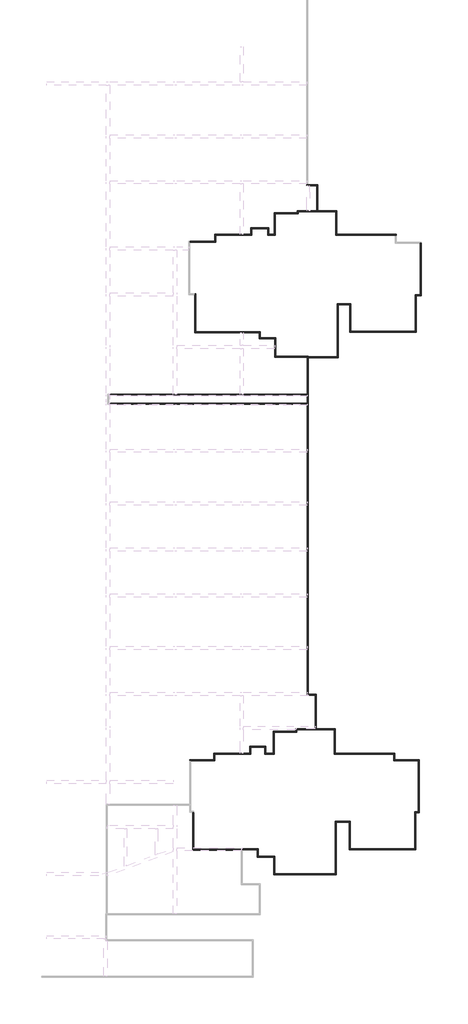
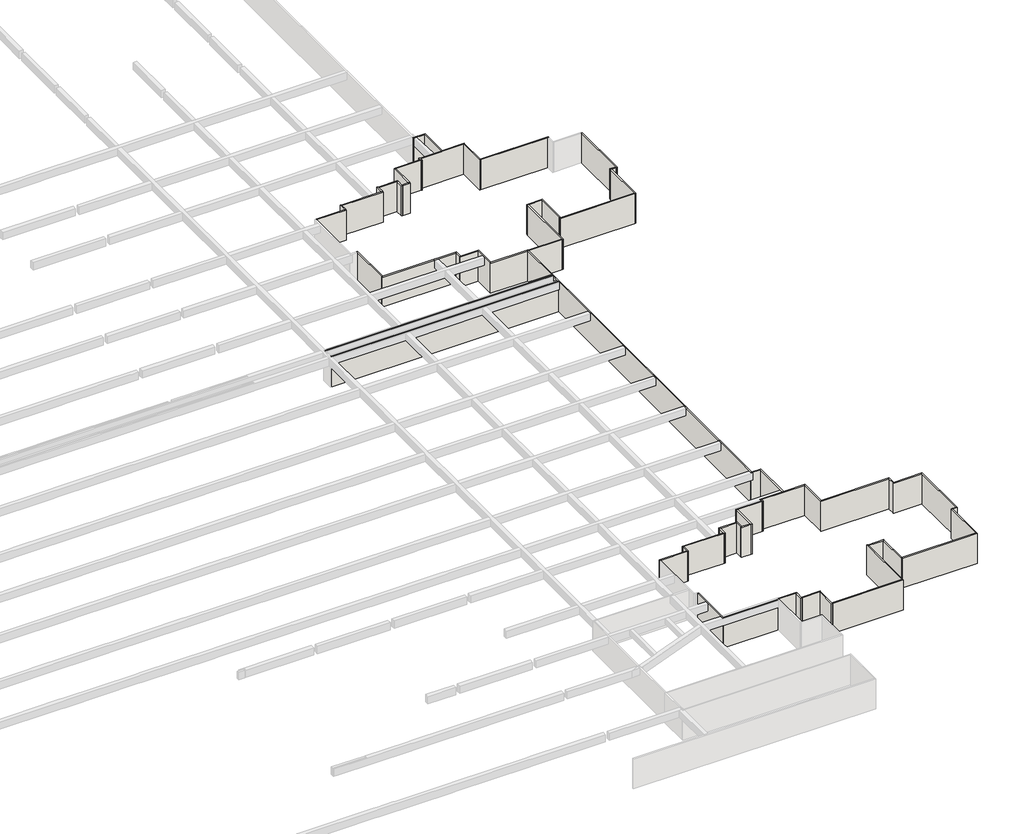
# One storey, part 5 of 14: 63 walls.
"""IFC4 building model written with IfcOpenShell, lengths in millimetres."""

from ifc_helpers import new_model, si_unit, origin, origin_with_axes, place, context, project, spatial, polyline, outline, extrude, faceted_brep, element, save

model = new_model("IFC4")

# Units and contexts
model_context = context("Model", 3, world=origin())
ifc_project = project(units=[si_unit("LENGTHUNIT", "METRE", prefix="MILLI")], contexts=[model_context])

# Site, building, storey
site = spatial("IfcSite", under=ifc_project)
building = spatial("IfcBuilding", under=site)
storey = spatial("IfcBuildingStorey", under=building, Name="户型图", Elevation=0.0)

# Walls
placement = place(None, origin())
element("IfcWall", 1, ObjectType="所有墙体", at=placement, inside=storey, context=model_context, shape_type="Brep", body=[
    faceted_brep([(-506007.6529952, -182584.2232736, 0.0), (-504227.6529952, -182584.2232736, 0.0), (-504107.6529952, -182584.2232736, 0.0), (-504107.6529952, -182584.2232736, 3300.0), (-504227.6529952, -182584.2232736, 3300.0), (-506007.6529952, -182584.2232736, 3300.0), (-506007.6529952, -182464.2232736, 0.0), (-506007.6529952, -182464.2232736, 3300.0), (-504107.6529952, -182464.2232736, 3300.0), (-504107.6529952, -182464.2232736, 0.0)], [[[0, 1, 2, 3, 4, 5]], [[6, 7, 8, 9]], [[2, 1, 0, 6, 9]], [[5, 4, 3, 8, 7]], [[0, 5, 7, 6]], [[3, 2, 9, 8]]]),
])
element("IfcWall", 2, ObjectType="所有墙体", at=placement, inside=storey, context=model_context, shape_type="Brep", body=[
    faceted_brep([(-504227.6529952, -182584.2232736, 0.0), (-504227.6529952, -183484.2232736, 0.0), (-504227.6529952, -183484.2232736, 3300.0), (-504227.6529952, -182584.2232736, 3300.0), (-504107.6529952, -182584.2232736, 0.0), (-504107.6529952, -182584.2232736, 3300.0), (-504107.6529952, -183364.2232736, 3300.0), (-504107.6529952, -183484.2232736, 3300.0), (-504107.6529952, -183484.2232736, 0.0), (-504107.6529952, -183364.2232736, 0.0)], [[[0, 1, 2, 3]], [[4, 5, 6, 7, 8, 9]], [[1, 0, 4, 9, 8]], [[3, 2, 7, 6, 5]], [[0, 3, 5, 4]], [[2, 1, 8, 7]]]),
])
element("IfcWall", 3, ObjectType="所有墙体", at=placement, inside=storey, context=model_context, shape_type="Brep", body=[
    faceted_brep([(-504107.6529952, -183484.2232736, 0.0), (-502261.0765844, -183484.2232736, 0.0), (-502141.0765844, -183484.2232736, 0.0), (-502141.0765844, -183484.2232736, 3300.0), (-502261.0765844, -183484.2232736, 3300.0), (-504107.6529952, -183484.2232736, 3300.0), (-504107.6529952, -183364.2232736, 0.0), (-504107.6529952, -183364.2232736, 3300.0), (-502141.0765844, -183364.2232736, 3300.0), (-502141.0765844, -183364.2232736, 0.0)], [[[0, 1, 2, 3, 4, 5]], [[6, 7, 8, 9]], [[2, 1, 0, 6, 9]], [[5, 4, 3, 8, 7]], [[0, 5, 7, 6]], [[3, 2, 9, 8]]]),
])
element("IfcWall", 4, ObjectType="所有墙体", at=placement, inside=storey, context=model_context, shape_type="Brep", body=[
    faceted_brep([(-502261.0765844, -183484.2232736, 0.0), (-502261.0765844, -185595.7483417, 0.0), (-502261.0765844, -185595.7483417, 3300.0), (-502261.0765844, -183484.2232736, 3300.0), (-502141.0765844, -183484.2232736, 0.0), (-502141.0765844, -183484.2232736, 3300.0), (-502141.0765844, -185475.7483417, 3300.0), (-502141.0765844, -185595.7483417, 3300.0), (-502141.0765844, -185595.7483417, 0.0), (-502141.0765844, -185475.7483417, 0.0)], [[[0, 1, 2, 3]], [[4, 5, 6, 7, 8, 9]], [[1, 0, 4, 9, 8]], [[3, 2, 7, 6, 5]], [[0, 3, 5, 4]], [[2, 1, 8, 7]]]),
])
element("IfcWall", 5, ObjectType="所有墙体", at=placement, inside=storey, context=model_context, shape_type="Brep", body=[
    faceted_brep([(-502141.0765844, -185595.7483417, 0.0), (-494747.3304181, -185595.7483417, 0.0), (-494747.3304181, -185595.7483417, 3300.0), (-502141.0765844, -185595.7483417, 3300.0), (-502141.0765844, -185475.7483417, 0.0), (-502141.0765844, -185475.7483417, 3300.0), (-494867.3304181, -185475.7483417, 3300.0), (-494747.3304181, -185475.7483417, 3300.0), (-494747.3304181, -185475.7483417, 0.0), (-494867.3304181, -185475.7483417, 0.0)], [[[0, 1, 2, 3]], [[4, 5, 6, 7, 8, 9]], [[1, 0, 4, 9, 8]], [[3, 2, 7, 6, 5]], [[0, 3, 5, 4]], [[2, 1, 8, 7]]]),
])
element("IfcWall", 6, ObjectType="所有墙体", at=placement, inside=storey, context=model_context, shape_type="Brep", body=[
    faceted_brep([(-494747.3304181, -185475.7483417, 0.0), (-494747.3304181, -179317.7334824, 0.0), (-494747.3304181, -179197.7334824, 0.0), (-494747.3304181, -179197.7334824, 3300.0), (-494747.3304181, -179317.7334824, 3300.0), (-494747.3304181, -185475.7483417, 3300.0), (-494867.3304181, -185475.7483417, 0.0), (-494867.3304181, -185475.7483417, 3300.0), (-494867.3304181, -179197.7334824, 3300.0), (-494867.3304181, -179197.7334824, 0.0)], [[[0, 1, 2, 3, 4, 5]], [[6, 7, 8, 9]], [[2, 1, 0, 6, 9]], [[5, 4, 3, 8, 7]], [[0, 5, 7, 6]], [[3, 2, 9, 8]]]),
])
element("IfcWall", 7, ObjectType="所有墙体", at=placement, inside=storey, context=model_context, shape_type="Brep", body=[
    faceted_brep([(-494747.3304181, -179317.7334824, 0.0), (-493248.6319968, -179317.7334824, 0.0), (-493128.6319968, -179317.7334824, 0.0), (-493128.6319968, -179317.7334824, 3300.0), (-493248.6319968, -179317.7334824, 3300.0), (-494747.3304181, -179317.7334824, 3300.0), (-494747.3304181, -179197.7334824, 0.0), (-494747.3304181, -179197.7334824, 3300.0), (-493128.6319968, -179197.7334824, 3300.0), (-493128.6319968, -179197.7334824, 0.0)], [[[0, 1, 2, 3, 4, 5]], [[6, 7, 8, 9]], [[2, 1, 0, 6, 9]], [[5, 4, 3, 8, 7]], [[0, 5, 7, 6]], [[3, 2, 9, 8]]]),
])
element("IfcWall", 8, ObjectType="所有墙体", at=placement, inside=storey, context=model_context, shape_type="Brep", body=[
    faceted_brep([(-493248.6319968, -179317.7334824, 0.0), (-493248.6319968, -182584.2232736, 0.0), (-493248.6319968, -182584.2232736, 3300.0), (-493248.6319968, -179317.7334824, 3300.0), (-493128.6319968, -179317.7334824, 0.0), (-493128.6319968, -179317.7334824, 3300.0), (-493128.6319968, -182464.2232736, 3300.0), (-493128.6319968, -182584.2232736, 3300.0), (-493128.6319968, -182584.2232736, 0.0), (-493128.6319968, -182464.2232736, 0.0)], [[[0, 1, 2, 3]], [[4, 5, 6, 7, 8, 9]], [[1, 0, 4, 9, 8]], [[3, 2, 7, 6, 5]], [[0, 3, 5, 4]], [[2, 1, 8, 7]]]),
])
element("IfcWall", 9, ObjectType="所有墙体", at=placement, inside=storey, context=model_context, shape_type="Brep", body=[
    faceted_brep([(-493128.6319968, -182584.2232736, 0.0), (-485288.3223724, -182584.2232736, 0.0), (-485288.3223724, -182584.2232736, 3300.0), (-493128.6319968, -182584.2232736, 3300.0), (-493128.6319968, -182464.2232736, 0.0), (-493128.6319968, -182464.2232736, 3300.0), (-485408.3223724, -182464.2232736, 3300.0), (-485288.3223724, -182464.2232736, 3300.0), (-485288.3223724, -182464.2232736, 0.0), (-485408.3223724, -182464.2232736, 0.0)], [[[0, 1, 2, 3]], [[4, 5, 6, 7, 8, 9]], [[1, 0, 4, 9, 8]], [[3, 2, 7, 6, 5]], [[0, 3, 5, 4]], [[2, 1, 8, 7]]]),
])
element("IfcWall", 10, ObjectType="所有墙体", at=placement, inside=storey, context=model_context, shape_type="Brep", body=[
    faceted_brep([(-485288.3223724, -182464.2232736, 0.0), (-485288.3223724, -178145.8900452, 0.0), (-485288.3223724, -178025.8900452, 0.0), (-485288.3223724, -178025.8900452, 3300.0), (-485288.3223724, -178145.8900452, 3300.0), (-485288.3223724, -182464.2232736, 3300.0), (-485408.3223724, -182464.2232736, 0.0), (-485408.3223724, -182464.2232736, 3300.0), (-485408.3223724, -178025.8900452, 3300.0), (-485408.3223724, -178025.8900452, 0.0)], [[[0, 1, 2, 3, 4, 5]], [[6, 7, 8, 9]], [[2, 1, 0, 6, 9]], [[5, 4, 3, 8, 7]], [[0, 5, 7, 6]], [[3, 2, 9, 8]]]),
])
element("IfcWall", 11, ObjectType="所有墙体", at=placement, inside=storey, context=model_context, shape_type="Brep", body=[
    faceted_brep([(-485288.3223724, -178145.8900452, 0.0), (-484825.1063307, -178145.8900452, 0.0), (-484825.1063307, -178145.8900452, 3300.0), (-485288.3223724, -178145.8900452, 3300.0), (-485288.3223724, -178025.8900452, 0.0), (-485288.3223724, -178025.8900452, 3300.0), (-484945.1063307, -178025.8900452, 3300.0), (-484825.1063307, -178025.8900452, 3300.0), (-484825.1063307, -178025.8900452, 0.0), (-484945.1063307, -178025.8900452, 0.0)], [[[0, 1, 2, 3]], [[4, 5, 6, 7, 8, 9]], [[1, 0, 4, 9, 8]], [[3, 2, 7, 6, 5]], [[0, 3, 5, 4]], [[2, 1, 8, 7]]]),
])
element("IfcWall", 12, ObjectType="所有墙体", at=placement, inside=storey, context=model_context, shape_type="Brep", body=[
    faceted_brep([(-484825.1063307, -178025.8900452, 0.0), (-484825.1063307, -171827.2416788, 0.0), (-484825.1063307, -171827.2416788, 3300.0), (-484825.1063307, -178025.8900452, 3300.0), (-484945.1063307, -178025.8900452, 0.0), (-484945.1063307, -178025.8900452, 3300.0), (-484945.1063307, -171947.2416788, 3300.0), (-484945.1063307, -171827.2416788, 3300.0), (-484945.1063307, -171827.2416788, 0.0), (-484945.1063307, -171947.2416788, 0.0)], [[[0, 1, 2, 3]], [[4, 5, 6, 7, 8, 9]], [[1, 0, 4, 9, 8]], [[3, 2, 7, 6, 5]], [[0, 3, 5, 4]], [[2, 1, 8, 7]]]),
])
element("IfcWall", 13, ObjectType="所有墙体", at=placement, inside=storey, context=model_context, shape_type="Brep", body=[
    faceted_brep([(-484945.1063307, -171827.2416788, 0.0), (-487806.6646743, -171827.2416788, 0.0), (-487926.6646743, -171827.2416788, 0.0), (-487926.6646743, -171827.2416788, 3300.0), (-487806.6646743, -171827.2416788, 3300.0), (-484945.1063307, -171827.2416788, 3300.0), (-484945.1063307, -171947.2416788, 0.0), (-484945.1063307, -171947.2416788, 3300.0), (-487926.6646743, -171947.2416788, 3300.0), (-487926.6646743, -171947.2416788, 0.0)], [[[0, 1, 2, 3, 4, 5]], [[6, 7, 8, 9]], [[2, 1, 0, 6, 9]], [[5, 4, 3, 8, 7]], [[0, 5, 7, 6]], [[3, 2, 9, 8]]]),
])
element("IfcWall", 14, ObjectType="所有墙体", at=placement, inside=storey, context=model_context, shape_type="Brep", body=[
    faceted_brep([(-487806.6646743, -171827.2416788, 0.0), (-487806.6646743, -171018.3612758, 0.0), (-487806.6646743, -171018.3612758, 3300.0), (-487806.6646743, -171827.2416788, 3300.0), (-487926.6646743, -171827.2416788, 0.0), (-487926.6646743, -171827.2416788, 3300.0), (-487926.6646743, -171138.3612758, 3300.0), (-487926.6646743, -171018.3612758, 3300.0), (-487926.6646743, -171018.3612758, 0.0), (-487926.6646743, -171138.3612758, 0.0)], [[[0, 1, 2, 3]], [[4, 5, 6, 7, 8, 9]], [[1, 0, 4, 9, 8]], [[3, 2, 7, 6, 5]], [[0, 3, 5, 4]], [[2, 1, 8, 7]]]),
])
element("IfcWall", 15, ObjectType="所有墙体", at=placement, inside=storey, context=model_context, shape_type="Brep", body=[
    faceted_brep([(-487926.6646743, -171018.3612758, 0.0), (-494904.2878989, -171018.3612758, 0.0), (-495024.2878989, -171018.3612758, 0.0), (-495024.2878989, -171018.3612758, 3300.0), (-494904.2878989, -171018.3612758, 3300.0), (-487926.6646743, -171018.3612758, 3300.0), (-487926.6646743, -171138.3612758, 0.0), (-487926.6646743, -171138.3612758, 3300.0), (-495024.2878989, -171138.3612758, 3300.0), (-495024.2878989, -171138.3612758, 0.0)], [[[0, 1, 2, 3, 4, 5]], [[6, 7, 8, 9]], [[2, 1, 0, 6, 9]], [[5, 4, 3, 8, 7]], [[0, 5, 7, 6]], [[3, 2, 9, 8]]]),
])
element("IfcWall", 16, ObjectType="所有墙体", at=placement, inside=storey, context=model_context, shape_type="Brep", body=[
    faceted_brep([(-494904.2878989, -171018.3612758, 0.0), (-494904.2878989, -168097.2169847, 0.0), (-494904.2878989, -168097.2169847, 3300.0), (-494904.2878989, -171018.3612758, 3300.0), (-495024.2878989, -171018.3612758, 0.0), (-495024.2878989, -171018.3612758, 3300.0), (-495024.2878989, -168217.2169847, 3300.0), (-495024.2878989, -168097.2169847, 3300.0), (-495024.2878989, -168097.2169847, 0.0), (-495024.2878989, -168217.2169847, 0.0)], [[[0, 1, 2, 3]], [[4, 5, 6, 7, 8, 9]], [[1, 0, 4, 9, 8]], [[3, 2, 7, 6, 5]], [[0, 3, 5, 4]], [[2, 1, 8, 7]]]),
])
element("IfcWall", 17, ObjectType="所有墙体", at=placement, inside=storey, context=model_context, shape_type="Brep", body=[
    faceted_brep([(-495024.2878989, -168097.2169847, 0.0), (-497157.6529954, -168097.2169847, 0.0), (-497277.6529954, -168097.2169847, 0.0), (-499504.2878989, -168097.2169847, 0.0), (-499504.2878989, -168097.2169847, 3300.0), (-497277.6529954, -168097.2169847, 3300.0), (-497157.6529954, -168097.2169847, 3300.0), (-495024.2878989, -168097.2169847, 3300.0), (-495024.2878989, -168217.2169847, 0.0), (-495024.2878989, -168217.2169847, 3300.0), (-499504.2878989, -168217.2169847, 3300.0), (-499504.2878989, -168217.2169847, 0.0)], [[[0, 1, 2, 3, 4, 5, 6, 7]], [[8, 9, 10, 11]], [[3, 2, 1, 0, 8, 11]], [[7, 6, 5, 4, 10, 9]], [[0, 7, 9, 8]], [[4, 3, 11, 10]]]),
])
element("IfcWall", 18, ObjectType="所有墙体", at=placement, inside=storey, context=model_context, shape_type="Brep", body=[
    faceted_brep([(-499624.2878989, -168097.2169847, 0.0), (-499624.2878989, -168383.5229446, 0.0), (-499624.2878989, -168503.5229446, 0.0), (-499624.2878989, -168503.5229446, 3300.0), (-499624.2878989, -168383.5229446, 3300.0), (-499624.2878989, -168200.507479, 3300.0), (-499624.2878989, -168097.2169847, 3300.0), (-499624.2878989, -168097.2169847, 2500.0), (-499504.2878989, -168097.2169847, 0.0), (-499504.2878989, -168097.2169847, 3300.0), (-499504.2878989, -168217.2169847, 3300.0), (-499504.2878989, -168503.5229446, 3300.0), (-499504.2878989, -168503.5229446, 0.0), (-499504.2878989, -168217.2169847, 0.0)], [[[0, 1, 2, 3, 4, 5, 6, 7]], [[8, 9, 10, 11, 12, 13]], [[2, 1, 0, 8, 13, 12]], [[6, 5, 4, 3, 11, 10, 9]], [[0, 7, 6, 9, 8]], [[3, 2, 12, 11]]]),
])
element("IfcWall", 19, ObjectType="所有墙体", at=placement, inside=storey, context=model_context, shape_type="Brep", body=[
    faceted_brep([(-499624.2878989, -168383.5229446, 0.0), (-502316.4756763, -168383.5229446, 0.0), (-502316.4756763, -168383.5229446, 3300.0), (-499624.2878989, -168383.5229446, 3300.0), (-499624.2878989, -168503.5229446, 0.0), (-499624.2878989, -168503.5229446, 3300.0), (-502196.4756763, -168503.5229446, 3300.0), (-502316.4756763, -168503.5229446, 3300.0), (-502316.4756763, -168503.5229446, 0.0), (-502196.4756763, -168503.5229446, 0.0)], [[[0, 1, 2, 3]], [[4, 5, 6, 7, 8, 9]], [[1, 0, 4, 9, 8]], [[3, 2, 7, 6, 5]], [[0, 3, 5, 4]], [[2, 1, 8, 7]]]),
])
element("IfcWall", 20, ObjectType="所有墙体", at=placement, inside=storey, context=model_context, shape_type="Brep", body=[
    faceted_brep([(-502316.4756763, -168503.5229446, 0.0), (-502316.4756763, -171018.3612758, 0.0), (-502316.4756763, -171138.3612758, 0.0), (-502316.4756763, -171138.3612758, 3300.0), (-502316.4756763, -171018.3612758, 3300.0), (-502316.4756763, -168503.5229446, 3300.0), (-502196.4756763, -168503.5229446, 0.0), (-502196.4756763, -168503.5229446, 3300.0), (-502196.4756763, -171138.3612758, 3300.0), (-502196.4756763, -171138.3612758, 0.0)], [[[0, 1, 2, 3, 4, 5]], [[6, 7, 8, 9]], [[2, 1, 0, 6, 9]], [[5, 4, 3, 8, 7]], [[0, 5, 7, 6]], [[3, 2, 9, 8]]]),
])
element("IfcWall", 21, ObjectType="所有墙体", at=placement, inside=storey, context=model_context, shape_type="Brep", body=[
    faceted_brep([(-502316.4756763, -171018.3612758, 0.0), (-503204.3247875, -171018.3612758, 0.0), (-503324.3247875, -171018.3612758, 0.0), (-503324.3247875, -171018.3612758, 3300.0), (-503204.3247875, -171018.3612758, 3300.0), (-502316.4756763, -171018.3612758, 3300.0), (-502316.4756763, -171138.3612758, 0.0), (-502316.4756763, -171138.3612758, 3300.0), (-503324.3247875, -171138.3612758, 3300.0), (-503324.3247875, -171138.3612758, 0.0)], [[[0, 1, 2, 3, 4, 5]], [[6, 7, 8, 9]], [[2, 1, 0, 6, 9]], [[5, 4, 3, 8, 7]], [[0, 5, 7, 6]], [[3, 2, 9, 8]]]),
])
element("IfcWall", 22, ObjectType="所有墙体", at=placement, inside=storey, context=model_context, shape_type="Brep", body=[
    faceted_brep([(-503204.3247875, -171018.3612758, 0.0), (-503204.3247875, -170172.5149791, 0.0), (-503204.3247875, -170172.5149791, 3300.0), (-503204.3247875, -171018.3612758, 3300.0), (-503324.3247875, -171018.3612758, 0.0), (-503324.3247875, -171018.3612758, 3300.0), (-503324.3247875, -170292.5149791, 3300.0), (-503324.3247875, -170172.5149791, 3300.0), (-503324.3247875, -170172.5149791, 0.0), (-503324.3247875, -170292.5149791, 0.0)], [[[0, 1, 2, 3]], [[4, 5, 6, 7, 8, 9]], [[1, 0, 4, 9, 8]], [[3, 2, 7, 6, 5]], [[0, 3, 5, 4]], [[2, 1, 8, 7]]]),
])
element("IfcWall", 23, ObjectType="所有墙体", at=placement, inside=storey, context=model_context, shape_type="Brep", body=[
    faceted_brep([(-503324.3247875, -170172.5149791, 0.0), (-505121.8144656, -170172.5149791, 0.0), (-505121.8144656, -170172.5149791, 3300.0), (-503324.3247875, -170172.5149791, 3300.0), (-503324.3247875, -170292.5149791, 0.0), (-503324.3247875, -170292.5149791, 3300.0), (-505001.8144656, -170292.5149791, 3300.0), (-505121.8144656, -170292.5149791, 3300.0), (-505121.8144656, -170292.5149791, 0.0), (-505001.8144656, -170292.5149791, 0.0)], [[[0, 1, 2, 3]], [[4, 5, 6, 7, 8, 9]], [[1, 0, 4, 9, 8]], [[3, 2, 7, 6, 5]], [[0, 3, 5, 4]], [[2, 1, 8, 7]]]),
])
element("IfcWall", 24, ObjectType="所有墙体", at=placement, inside=storey, context=model_context, shape_type="Brep", body=[
    faceted_brep([(-505121.8144656, -170292.5149791, 0.0), (-505121.8144656, -171018.3612758, 0.0), (-505121.8144656, -171138.3612758, 0.0), (-505121.8144656, -171138.3612758, 3300.0), (-505121.8144656, -171018.3612758, 3300.0), (-505121.8144656, -170292.5149791, 3300.0), (-505001.8144656, -170292.5149791, 0.0), (-505001.8144656, -170292.5149791, 3300.0), (-505001.8144656, -171138.3612758, 3300.0), (-505001.8144656, -171138.3612758, 0.0)], [[[0, 1, 2, 3, 4, 5]], [[6, 7, 8, 9]], [[2, 1, 0, 6, 9]], [[5, 4, 3, 8, 7]], [[0, 5, 7, 6]], [[3, 2, 9, 8]]]),
])
element("IfcWall", 25, ObjectType="所有墙体", at=placement, inside=storey, context=model_context, shape_type="Brep", body=[
    faceted_brep([(-505121.8144656, -171018.3612758, 0.0), (-509424.3517261, -171018.3612758, 0.0), (-509424.3517261, -171018.3612758, 3300.0), (-505121.8144656, -171018.3612758, 3300.0), (-505121.8144656, -171138.3612758, 0.0), (-505121.8144656, -171138.3612758, 3300.0), (-509304.3517261, -171138.3612758, 3300.0), (-509424.3517261, -171138.3612758, 3300.0), (-509424.3517261, -171138.3612758, 0.0), (-509304.3517261, -171138.3612758, 0.0)], [[[0, 1, 2, 3]], [[4, 5, 6, 7, 8, 9]], [[1, 0, 4, 9, 8]], [[3, 2, 7, 6, 5]], [[0, 3, 5, 4]], [[2, 1, 8, 7]]]),
])
element("IfcWall", 26, ObjectType="所有墙体", at=placement, inside=storey, context=model_context, shape_type="Brep", body=[
    faceted_brep([(-509424.3517261, -171138.3612758, 0.0), (-509424.3517261, -171827.2416788, 0.0), (-509424.3517261, -171947.2416788, 0.0), (-509424.3517261, -171947.2416788, 3300.0), (-509424.3517261, -171827.2416788, 3300.0), (-509424.3517261, -171138.3612758, 3300.0), (-509304.3517261, -171138.3612758, 0.0), (-509304.3517261, -171138.3612758, 3300.0), (-509304.3517261, -171947.2416788, 3300.0), (-509304.3517261, -171947.2416788, 0.0)], [[[0, 1, 2, 3, 4, 5]], [[6, 7, 8, 9]], [[2, 1, 0, 6, 9]], [[5, 4, 3, 8, 7]], [[0, 5, 7, 6]], [[3, 2, 9, 8]]]),
])
element("IfcWall", 27, ObjectType="所有墙体", at=placement, inside=storey, context=model_context, shape_type="Brep", body=[
    faceted_brep([(-509424.3517261, -171827.2416788, 0.0), (-512303.9222774, -171827.2416788, 0.0), (-512303.9222774, -171827.2416788, 3300.0), (-509424.3517261, -171827.2416788, 3300.0), (-509424.3517261, -171947.2416788, 0.0), (-509424.3517261, -171947.2416788, 3300.0), (-512183.9222774, -171947.2416788, 3300.0), (-512303.9222774, -171947.2416788, 3300.0), (-512303.9222774, -171947.2416788, 0.0), (-512183.9222774, -171947.2416788, 0.0)], [[[0, 1, 2, 3]], [[4, 5, 6, 7, 8, 9]], [[1, 0, 4, 9, 8]], [[3, 2, 7, 6, 5]], [[0, 3, 5, 4]], [[2, 1, 8, 7]]]),
])
element("IfcWall", 28, ObjectType="所有墙体", at=placement, inside=storey, context=model_context, shape_type="Brep", body=[
    faceted_brep([(-497157.6529954, -168097.2169847, 0.0), (-497157.6529954, -163999.4327531, 0.0), (-497157.6529954, -163999.4327531, 3300.0), (-497157.6529954, -168097.2169847, 3300.0), (-497277.6529954, -168097.2169847, 0.0), (-497277.6529954, -168097.2169847, 3300.0), (-497277.6529954, -164119.4327531, 3300.0), (-497277.6529954, -163999.4327531, 3300.0), (-497277.6529954, -163999.4327531, 0.0), (-497277.6529954, -164119.4327531, 0.0)], [[[0, 1, 2, 3]], [[4, 5, 6, 7, 8, 9]], [[1, 0, 4, 9, 8]], [[3, 2, 7, 6, 5]], [[0, 3, 5, 4]], [[2, 1, 8, 7]]]),
])
element("IfcWall", 29, ObjectType="所有墙体", at=placement, inside=storey, context=model_context, shape_type="Brep", body=[
    faceted_brep([(-497277.6529954, -163999.4327531, 0.0), (-498107.6529954, -163999.4327531, 0.0), (-498227.6529954, -163999.4327531, 0.0), (-498227.6529954, -163999.4327531, 3300.0), (-498107.6529954, -163999.4327531, 3300.0), (-497277.6529954, -163999.4327531, 3300.0), (-497277.6529954, -164119.4327531, 0.0), (-497277.6529954, -164119.4327531, 3300.0), (-498107.6529954, -164119.4327531, 3300.0), (-498227.6529954, -164119.4327531, 3300.0), (-498227.6529954, -164119.4327531, 2500.0), (-498227.6529954, -164119.4327531, 0.0)], [[[0, 1, 2, 3, 4, 5]], [[6, 7, 8, 9, 10, 11]], [[2, 1, 0, 6, 11]], [[5, 4, 3, 9, 8, 7]], [[0, 5, 7, 6]], [[3, 2, 11, 10, 9]]]),
])
element("IfcWall", 30, ObjectType="所有墙体", at=placement, inside=storey, context=model_context, shape_type="Brep", body=[
    faceted_brep([(-498107.6529954, -163999.4327531, 0.0), (-498107.6529954, -123717.5126628, 0.0), (-498107.6529954, -123597.5126628, 0.0), (-498107.6529954, -123587.4825125, 0.0), (-498107.6529954, -123587.4825125, 3300.0), (-498107.6529954, -123597.5126628, 3300.0), (-498107.6529954, -123717.5126628, 3300.0), (-498107.6529954, -151959.4327531, 3300.0), (-498107.6529954, -152359.4327531, 3300.0), (-498107.6529954, -163999.4327531, 3300.0), (-498227.6529954, -163999.4327531, 0.0), (-498227.6529954, -163999.4327531, 3300.0), (-498227.6529954, -152359.4327531, 3300.0), (-498227.6529954, -151959.4327531, 3300.0), (-498227.6529954, -129294.4327531, 3300.0), (-498227.6529954, -129174.4327531, 3300.0), (-498227.6529954, -128219.4327532, 3300.0), (-498227.6529954, -128099.4327532, 3300.0), (-498227.6529954, -123707.4825125, 3300.0), (-498227.6529954, -123587.4825125, 3300.0), (-498227.6529954, -123587.4825125, 0.0), (-498227.6529954, -123707.4825125, 0.0), (-498227.6529954, -128099.4327532, 0.0), (-498227.6529954, -128219.4327532, 0.0), (-498227.6529954, -129174.4327531, 0.0), (-498227.6529954, -129294.4327531, 0.0)], [[[0, 1, 2, 3, 4, 5, 6, 7, 8, 9]], [[10, 11, 12, 13, 14, 15, 16, 17, 18, 19, 20, 21, 22, 23, 24, 25]], [[3, 2, 1, 0, 10, 25, 24, 23, 22, 21, 20]], [[9, 8, 7, 6, 5, 4, 19, 18, 17, 16, 15, 14, 13, 12, 11]], [[0, 9, 11, 10]], [[4, 3, 20, 19]]]),
])
element("IfcWall", 31, ObjectType="所有墙体", at=placement, inside=storey, context=model_context, shape_type="Brep", body=[
    faceted_brep([(-498227.6529954, -123587.4825125, 0.0), (-502007.6529954, -123587.4825125, 0.0), (-502127.6529954, -123587.4825125, 0.0), (-502127.6529954, -123587.4825125, 3300.0), (-502007.6529954, -123587.4825125, 3300.0), (-498227.6529954, -123587.4825125, 3300.0), (-498227.6529954, -123707.4825125, 0.0), (-498227.6529954, -123707.4825125, 3300.0), (-502127.6529954, -123707.4825125, 3300.0), (-502127.6529954, -123707.4825125, 0.0)], [[[0, 1, 2, 3, 4, 5]], [[6, 7, 8, 9]], [[2, 1, 0, 6, 9]], [[5, 4, 3, 8, 7]], [[0, 5, 7, 6]], [[3, 2, 9, 8]]]),
])
element("IfcWall", 32, ObjectType="所有墙体", at=placement, inside=storey, context=model_context, shape_type="Brep", body=[
    faceted_brep([(-502007.6529954, -123587.4825125, 0.0), (-502007.6529954, -121375.8614811, 0.0), (-502007.6529954, -121375.8614811, 3300.0), (-502007.6529954, -123587.4825125, 3300.0), (-502127.6529954, -123587.4825125, 0.0), (-502127.6529954, -123587.4825125, 3300.0), (-502127.6529954, -121495.8614811, 3300.0), (-502127.6529954, -121375.8614811, 3300.0), (-502127.6529954, -121375.8614811, 0.0), (-502127.6529954, -121495.8614811, 0.0)], [[[0, 1, 2, 3]], [[4, 5, 6, 7, 8, 9]], [[1, 0, 4, 9, 8]], [[3, 2, 7, 6, 5]], [[0, 3, 5, 4]], [[2, 1, 8, 7]]]),
])
element("IfcWall", 33, ObjectType="所有墙体", at=placement, inside=storey, context=model_context, shape_type="Brep", body=[
    faceted_brep([(-502127.6529954, -121375.8614811, 0.0), (-503856.5299096, -121375.8614811, 0.0), (-503976.5299096, -121375.8614811, 0.0), (-503976.5299096, -121375.8614811, 3300.0), (-503856.5299096, -121375.8614811, 3300.0), (-502127.6529954, -121375.8614811, 3300.0), (-502127.6529954, -121495.8614811, 0.0), (-502127.6529954, -121495.8614811, 3300.0), (-503976.5299096, -121495.8614811, 3300.0), (-503976.5299096, -121495.8614811, 0.0)], [[[0, 1, 2, 3, 4, 5]], [[6, 7, 8, 9]], [[2, 1, 0, 6, 9]], [[5, 4, 3, 8, 7]], [[0, 5, 7, 6]], [[3, 2, 9, 8]]]),
])
element("IfcWall", 34, ObjectType="所有墙体", at=placement, inside=storey, context=model_context, shape_type="Brep", body=[
    faceted_brep([(-503856.5299096, -121375.8614811, 0.0), (-503856.5299096, -120620.3535812, 0.0), (-503856.5299096, -120620.3535812, 3300.0), (-503856.5299096, -121375.8614811, 3300.0), (-503976.5299096, -121375.8614811, 0.0), (-503976.5299096, -121375.8614811, 3300.0), (-503976.5299096, -120740.3535812, 3300.0), (-503976.5299096, -120620.3535812, 3300.0), (-503976.5299096, -120620.3535812, 0.0), (-503976.5299096, -120740.3535812, 0.0)], [[[0, 1, 2, 3]], [[4, 5, 6, 7, 8, 9]], [[1, 0, 4, 9, 8]], [[3, 2, 7, 6, 5]], [[0, 3, 5, 4]], [[2, 1, 8, 7]]]),
])
element("IfcWall", 35, ObjectType="所有墙体", at=placement, inside=storey, context=model_context, shape_type="Brep", body=[
    faceted_brep([(-503976.5299096, -120620.3535812, 0.0), (-511554.3146967, -120620.3535812, 0.0), (-511674.3146967, -120620.3535812, 0.0), (-511674.3146967, -120620.3535812, 3300.0), (-511554.3146967, -120620.3535812, 3300.0), (-503976.5299096, -120620.3535812, 3300.0), (-503976.5299096, -120740.3535812, 0.0), (-503976.5299096, -120740.3535812, 3300.0), (-511674.3146967, -120740.3535812, 3300.0), (-511674.3146967, -120740.3535812, 0.0)], [[[0, 1, 2, 3, 4, 5]], [[6, 7, 8, 9]], [[2, 1, 0, 6, 9]], [[5, 4, 3, 8, 7]], [[0, 5, 7, 6]], [[3, 2, 9, 8]]]),
])
element("IfcWall", 36, ObjectType="所有墙体", at=placement, inside=storey, context=model_context, shape_type="Brep", body=[
    faceted_brep([(-511554.3146967, -120620.3535812, 0.0), (-511554.3146967, -116097.5126628, 0.0), (-511554.3146967, -116097.5126628, 3300.0), (-511554.3146967, -120620.3535812, 3300.0), (-511674.3146967, -120620.3535812, 0.0), (-511674.3146967, -120620.3535812, 3300.0), (-511674.3146967, -116217.5126628, 3300.0), (-511674.3146967, -116097.5126628, 3300.0), (-511674.3146967, -116097.5126628, 0.0), (-511674.3146967, -116217.5126628, 0.0)], [[[0, 1, 2, 3]], [[4, 5, 6, 7, 8, 9]], [[1, 0, 4, 9, 8]], [[3, 2, 7, 6, 5]], [[0, 3, 5, 4]], [[2, 1, 8, 7]]]),
])
element("IfcWall", 37, ObjectType="所有墙体", at=placement, inside=storey, context=model_context, shape_type="Brep", body=[
    faceted_brep([(-512290.8523761, -109917.5126628, 0.0), (-509190.8523761, -109917.5126628, 0.0), (-509190.8523761, -109917.5126628, 3300.0), (-512290.8523761, -109917.5126628, 3300.0), (-512290.8523761, -109797.5126628, 0.0), (-512290.8523761, -109797.5126628, 3300.0), (-509310.8523761, -109797.5126628, 3300.0), (-509190.8523761, -109797.5126628, 3300.0), (-509190.8523761, -109797.5126628, 0.0), (-509310.8523761, -109797.5126628, 0.0)], [[[0, 1, 2, 3]], [[4, 5, 6, 7, 8, 9]], [[1, 0, 4, 9, 8]], [[3, 2, 7, 6, 5]], [[0, 3, 5, 4]], [[2, 1, 8, 7]]]),
])
element("IfcWall", 38, ObjectType="所有墙体", at=placement, inside=storey, context=model_context, shape_type="Brep", body=[
    faceted_brep([(-509190.8523761, -109797.5126628, 0.0), (-509190.8523761, -109117.5126628, 0.0), (-509190.8523761, -108997.5126628, 0.0), (-509190.8523761, -108997.5126628, 3300.0), (-509190.8523761, -109117.5126628, 3300.0), (-509190.8523761, -109797.5126628, 3300.0), (-509310.8523761, -109797.5126628, 0.0), (-509310.8523761, -109797.5126628, 3300.0), (-509310.8523761, -108997.5126628, 3300.0), (-509310.8523761, -108997.5126628, 0.0)], [[[0, 1, 2, 3, 4, 5]], [[6, 7, 8, 9]], [[2, 1, 0, 6, 9]], [[5, 4, 3, 8, 7]], [[0, 5, 7, 6]], [[3, 2, 9, 8]]]),
])
element("IfcWall", 39, ObjectType="所有墙体", at=placement, inside=storey, context=model_context, shape_type="Brep", body=[
    faceted_brep([(-509190.8523761, -109117.5126628, 0.0), (-504890.8523761, -109117.5126628, 0.0), (-504890.8523761, -109117.5126628, 3300.0), (-509190.8523761, -109117.5126628, 3300.0), (-509190.8523761, -108997.5126628, 0.0), (-509190.8523761, -108997.5126628, 3300.0), (-505010.8523761, -108997.5126628, 3300.0), (-504890.8523761, -108997.5126628, 3300.0), (-504890.8523761, -108997.5126628, 0.0), (-505010.8523761, -108997.5126628, 0.0)], [[[0, 1, 2, 3]], [[4, 5, 6, 7, 8, 9]], [[1, 0, 4, 9, 8]], [[3, 2, 7, 6, 5]], [[0, 3, 5, 4]], [[2, 1, 8, 7]]]),
])
element("IfcWall", 40, ObjectType="所有墙体", at=placement, inside=storey, context=model_context, shape_type="Brep", body=[
    faceted_brep([(-504890.8523761, -108997.5126628, 0.0), (-504890.8523761, -108317.5126628, 0.0), (-504890.8523761, -108197.5126628, 0.0), (-504890.8523761, -108197.5126628, 3300.0), (-504890.8523761, -108317.5126628, 3300.0), (-504890.8523761, -108997.5126628, 3300.0), (-505010.8523761, -108997.5126628, 0.0), (-505010.8523761, -108997.5126628, 3300.0), (-505010.8523761, -108197.5126628, 3300.0), (-505010.8523761, -108197.5126628, 0.0)], [[[0, 1, 2, 3, 4, 5]], [[6, 7, 8, 9]], [[2, 1, 0, 6, 9]], [[5, 4, 3, 8, 7]], [[0, 5, 7, 6]], [[3, 2, 9, 8]]]),
])
element("IfcWall", 41, ObjectType="所有墙体", at=placement, inside=storey, context=model_context, shape_type="Brep", body=[
    faceted_brep([(-504890.8523761, -108317.5126628, 0.0), (-502987.2905062, -108317.5126628, 0.0), (-502867.2905062, -108317.5126628, 0.0), (-502867.2905062, -108317.5126628, 3300.0), (-502987.2905062, -108317.5126628, 3300.0), (-504890.8523761, -108317.5126628, 3300.0), (-504890.8523761, -108197.5126628, 0.0), (-504890.8523761, -108197.5126628, 3300.0), (-502867.2905062, -108197.5126628, 3300.0), (-502867.2905062, -108197.5126628, 0.0)], [[[0, 1, 2, 3, 4, 5]], [[6, 7, 8, 9]], [[2, 1, 0, 6, 9]], [[5, 4, 3, 8, 7]], [[0, 5, 7, 6]], [[3, 2, 9, 8]]]),
])
element("IfcWall", 42, ObjectType="所有墙体", at=placement, inside=storey, context=model_context, shape_type="Brep", body=[
    faceted_brep([(-502987.2905062, -108317.5126628, 0.0), (-502987.2905062, -109117.5126628, 0.0), (-502987.2905062, -109117.5126628, 3300.0), (-502987.2905062, -108317.5126628, 3300.0), (-502867.2905062, -108317.5126628, 0.0), (-502867.2905062, -108317.5126628, 3300.0), (-502867.2905062, -108997.5126628, 3300.0), (-502867.2905062, -109117.5126628, 3300.0), (-502867.2905062, -109117.5126628, 0.0), (-502867.2905062, -108997.5126628, 0.0)], [[[0, 1, 2, 3]], [[4, 5, 6, 7, 8, 9]], [[1, 0, 4, 9, 8]], [[3, 2, 7, 6, 5]], [[0, 3, 5, 4]], [[2, 1, 8, 7]]]),
])
element("IfcWall", 43, ObjectType="所有墙体", at=placement, inside=storey, context=model_context, shape_type="Brep", body=[
    faceted_brep([(-502867.2905062, -109117.5126628, 0.0), (-502067.2905062, -109117.5126628, 0.0), (-502067.2905062, -109117.5126628, 3300.0), (-502867.2905062, -109117.5126628, 3300.0), (-502867.2905062, -108997.5126628, 0.0), (-502867.2905062, -108997.5126628, 3300.0), (-502187.2905062, -108997.5126628, 3300.0), (-502067.2905062, -108997.5126628, 3300.0), (-502067.2905062, -108997.5126628, 0.0), (-502187.2905062, -108997.5126628, 0.0)], [[[0, 1, 2, 3]], [[4, 5, 6, 7, 8, 9]], [[1, 0, 4, 9, 8]], [[3, 2, 7, 6, 5]], [[0, 3, 5, 4]], [[2, 1, 8, 7]]]),
])
element("IfcWall", 44, ObjectType="所有墙体", at=placement, inside=storey, context=model_context, shape_type="Brep", body=[
    faceted_brep([(-502067.2905062, -108997.5126628, 0.0), (-502067.2905062, -106517.5126628, 0.0), (-502067.2905062, -106397.5126628, 0.0), (-502067.2905062, -106397.5126628, 3300.0), (-502067.2905062, -106517.5126628, 3300.0), (-502067.2905062, -108997.5126628, 3300.0), (-502187.2905062, -108997.5126628, 0.0), (-502187.2905062, -108997.5126628, 3300.0), (-502187.2905062, -106397.5126628, 3300.0), (-502187.2905062, -106397.5126628, 0.0)], [[[0, 1, 2, 3, 4, 5]], [[6, 7, 8, 9]], [[2, 1, 0, 6, 9]], [[5, 4, 3, 8, 7]], [[0, 5, 7, 6]], [[3, 2, 9, 8]]]),
])
element("IfcWall", 45, ObjectType="所有墙体", at=placement, inside=storey, context=model_context, shape_type="SweptSolid", body=[
    extrude(outline(polyline([(-499431.9156201, -106517.5126628), (-502067.2905062, -106517.5126628), (-502067.2905062, -106397.5126628), (-499431.9156201, -106397.5126628), (-499431.9156201, -106517.5126628)])), origin_with_axes(), (0.0, 0.0, 1.0), 3300.0),
])
element("IfcWall", 46, ObjectType="所有墙体", at=placement, inside=storey, context=model_context, shape_type="Brep", body=[
    faceted_brep([(-499311.9156201, -106517.5126628, 0.0), (-499311.9156201, -106253.8197785, 0.0), (-499311.9156201, -106133.8197785, 0.0), (-499311.9156201, -106133.8197785, 3300.0), (-499311.9156201, -106253.8197785, 3300.0), (-499311.9156201, -106517.5126628, 3300.0), (-499431.9156201, -106517.5126628, 0.0), (-499431.9156201, -106517.5126628, 3300.0), (-499431.9156201, -106397.5126628, 3300.0), (-499431.9156201, -106133.8197785, 3300.0), (-499431.9156201, -106133.8197785, 0.0), (-499431.9156201, -106397.5126628, 0.0)], [[[0, 1, 2, 3, 4, 5]], [[6, 7, 8, 9, 10, 11]], [[2, 1, 0, 6, 11, 10]], [[5, 4, 3, 9, 8, 7]], [[0, 5, 7, 6]], [[3, 2, 10, 9]]]),
])
element("IfcWall", 47, ObjectType="所有墙体", at=placement, inside=storey, context=model_context, shape_type="Brep", body=[
    faceted_brep([(-499311.9156201, -106253.8197785, 0.0), (-494831.9156201, -106253.8197785, 0.0), (-494711.9156201, -106253.8197785, 0.0), (-494711.9156201, -106253.8197785, 3300.0), (-494831.9156201, -106253.8197785, 3300.0), (-499311.9156201, -106253.8197785, 3300.0), (-499311.9156201, -106133.8197785, 0.0), (-499311.9156201, -106133.8197785, 3300.0), (-497131.9156201, -106133.8197785, 3300.0), (-497011.9156201, -106133.8197785, 3300.0), (-494711.9156201, -106133.8197785, 3300.0), (-494711.9156201, -106133.8197785, 0.0), (-497011.9156201, -106133.8197785, 0.0), (-497131.9156201, -106133.8197785, 0.0)], [[[0, 1, 2, 3, 4, 5]], [[6, 7, 8, 9, 10, 11, 12, 13]], [[2, 1, 0, 6, 13, 12, 11]], [[5, 4, 3, 10, 9, 8, 7]], [[0, 5, 7, 6]], [[3, 2, 11, 10]]]),
])
element("IfcWall", 48, ObjectType="所有墙体", at=placement, inside=storey, context=model_context, shape_type="Brep", body=[
    faceted_brep([(-494831.9156201, -106253.8197785, 0.0), (-494831.9156201, -109117.5126628, 0.0), (-494831.9156201, -109117.5126628, 3300.0), (-494831.9156201, -106253.8197785, 3300.0), (-494711.9156201, -106253.8197785, 0.0), (-494711.9156201, -106253.8197785, 3300.0), (-494711.9156201, -108997.5126628, 3300.0), (-494711.9156201, -109117.5126628, 3300.0), (-494711.9156201, -109117.5126628, 0.0), (-494711.9156201, -108997.5126628, 0.0)], [[[0, 1, 2, 3]], [[4, 5, 6, 7, 8, 9]], [[1, 0, 4, 9, 8]], [[3, 2, 7, 6, 5]], [[0, 3, 5, 4]], [[2, 1, 8, 7]]]),
])
element("IfcWall", 49, ObjectType="所有墙体", at=placement, inside=storey, context=model_context, shape_type="Brep", body=[
    faceted_brep([(-494711.9156201, -109117.5126628, 0.0), (-487731.9156201, -109117.5126628, 0.0), (-487611.9156201, -109117.5126628, 0.0), (-487611.9156201, -109117.5126628, 3300.0), (-487731.9156201, -109117.5126628, 3300.0), (-494711.9156201, -109117.5126628, 3300.0), (-494711.9156201, -108997.5126628, 0.0), (-494711.9156201, -108997.5126628, 3300.0), (-487611.9156201, -108997.5126628, 3300.0), (-487611.9156201, -108997.5126628, 0.0)], [[[0, 1, 2, 3, 4, 5]], [[6, 7, 8, 9]], [[2, 1, 0, 6, 9]], [[5, 4, 3, 8, 7]], [[0, 5, 7, 6]], [[3, 2, 9, 8]]]),
])
element("IfcWall", 50, ObjectType="所有墙体", at=placement, inside=storey, context=model_context, shape_type="Brep", body=[
    faceted_brep([(-484731.9156201, -110017.5126628, 0.0), (-484731.9156201, -116197.5126628, 0.0), (-484731.9156201, -116317.5126628, 0.0), (-484731.9156201, -116317.5126628, 3300.0), (-484731.9156201, -116197.5126628, 3300.0), (-484731.9156201, -110017.5126628, 3300.0), (-484611.9156201, -110017.5126628, 0.0), (-484611.9156201, -110017.5126628, 3300.0), (-484611.9156201, -116317.5126628, 3300.0), (-484611.9156201, -116317.5126628, 0.0)], [[[0, 1, 2, 3, 4, 5]], [[6, 7, 8, 9]], [[2, 1, 0, 6, 9]], [[5, 4, 3, 8, 7]], [[0, 5, 7, 6]], [[3, 2, 9, 8]]]),
])
element("IfcWall", 51, ObjectType="所有墙体", at=placement, inside=storey, context=model_context, shape_type="Brep", body=[
    faceted_brep([(-484731.9156201, -116197.5126628, 0.0), (-485331.9156201, -116197.5126628, 0.0), (-485331.9156201, -116197.5126628, 3300.0), (-484731.9156201, -116197.5126628, 3300.0), (-484731.9156201, -116317.5126628, 0.0), (-484731.9156201, -116317.5126628, 3300.0), (-485211.9156201, -116317.5126628, 3300.0), (-485331.9156201, -116317.5126628, 3300.0), (-485331.9156201, -116317.5126628, 0.0), (-485211.9156201, -116317.5126628, 0.0)], [[[0, 1, 2, 3]], [[4, 5, 6, 7, 8, 9]], [[1, 0, 4, 9, 8]], [[3, 2, 7, 6, 5]], [[0, 3, 5, 4]], [[2, 1, 8, 7]]]),
])
element("IfcWall", 52, ObjectType="所有墙体", at=placement, inside=storey, context=model_context, shape_type="Brep", body=[
    faceted_brep([(-485331.9156201, -116317.5126628, 0.0), (-485331.9156201, -120597.5126628, 0.0), (-485331.9156201, -120717.5126628, 0.0), (-485331.9156201, -120717.5126628, 3300.0), (-485331.9156201, -120597.5126628, 3300.0), (-485331.9156201, -116317.5126628, 3300.0), (-485211.9156201, -116317.5126628, 0.0), (-485211.9156201, -116317.5126628, 3300.0), (-485211.9156201, -120717.5126628, 3300.0), (-485211.9156201, -120717.5126628, 0.0)], [[[0, 1, 2, 3, 4, 5]], [[6, 7, 8, 9]], [[2, 1, 0, 6, 9]], [[5, 4, 3, 8, 7]], [[0, 5, 7, 6]], [[3, 2, 9, 8]]]),
])
element("IfcWall", 53, ObjectType="所有墙体", at=placement, inside=storey, context=model_context, shape_type="Brep", body=[
    faceted_brep([(-485331.9156201, -120597.5126628, 0.0), (-493011.9156201, -120597.5126628, 0.0), (-493131.9156201, -120597.5126628, 0.0), (-493131.9156201, -120597.5126628, 3300.0), (-493011.9156201, -120597.5126628, 3300.0), (-485331.9156201, -120597.5126628, 3300.0), (-485331.9156201, -120717.5126628, 0.0), (-485331.9156201, -120717.5126628, 3300.0), (-493131.9156201, -120717.5126628, 3300.0), (-493131.9156201, -120717.5126628, 0.0)], [[[0, 1, 2, 3, 4, 5]], [[6, 7, 8, 9]], [[2, 1, 0, 6, 9]], [[5, 4, 3, 8, 7]], [[0, 5, 7, 6]], [[3, 2, 9, 8]]]),
])
element("IfcWall", 54, ObjectType="所有墙体", at=placement, inside=storey, context=model_context, shape_type="Brep", body=[
    faceted_brep([(-493011.9156201, -120597.5126628, 0.0), (-493011.9156201, -117297.5126628, 0.0), (-493011.9156201, -117297.5126628, 3300.0), (-493011.9156201, -120597.5126628, 3300.0), (-493131.9156201, -120597.5126628, 0.0), (-493131.9156201, -120597.5126628, 3300.0), (-493131.9156201, -117417.5126628, 3300.0), (-493131.9156201, -117297.5126628, 3300.0), (-493131.9156201, -117297.5126628, 0.0), (-493131.9156201, -117417.5126628, 0.0)], [[[0, 1, 2, 3]], [[4, 5, 6, 7, 8, 9]], [[1, 0, 4, 9, 8]], [[3, 2, 7, 6, 5]], [[0, 3, 5, 4]], [[2, 1, 8, 7]]]),
])
element("IfcWall", 55, ObjectType="所有墙体", at=placement, inside=storey, context=model_context, shape_type="Brep", body=[
    faceted_brep([(-493131.9156201, -117297.5126628, 0.0), (-494631.9156201, -117297.5126628, 0.0), (-494631.9156201, -117297.5126628, 3300.0), (-493131.9156201, -117297.5126628, 3300.0), (-493131.9156201, -117417.5126628, 0.0), (-493131.9156201, -117417.5126628, 3300.0), (-494511.9156201, -117417.5126628, 3300.0), (-494631.9156201, -117417.5126628, 3300.0), (-494631.9156201, -117417.5126628, 0.0), (-494511.9156201, -117417.5126628, 0.0)], [[[0, 1, 2, 3]], [[4, 5, 6, 7, 8, 9]], [[1, 0, 4, 9, 8]], [[3, 2, 7, 6, 5]], [[0, 3, 5, 4]], [[2, 1, 8, 7]]]),
])
element("IfcWall", 56, ObjectType="所有墙体", at=placement, inside=storey, context=model_context, shape_type="Brep", body=[
    faceted_brep([(-494631.9156201, -117417.5126628, 0.0), (-494631.9156201, -123597.5126628, 0.0), (-494631.9156201, -123717.5126628, 0.0), (-494631.9156201, -123717.5126628, 3300.0), (-494631.9156201, -123597.5126628, 3300.0), (-494631.9156201, -117417.5126628, 3300.0), (-494511.9156201, -117417.5126628, 0.0), (-494511.9156201, -117417.5126628, 3300.0), (-494511.9156201, -123717.5126628, 3300.0), (-494511.9156201, -123717.5126628, 0.0)], [[[0, 1, 2, 3, 4, 5]], [[6, 7, 8, 9]], [[2, 1, 0, 6, 9]], [[5, 4, 3, 8, 7]], [[0, 5, 7, 6]], [[3, 2, 9, 8]]]),
])
element("IfcWall", 57, ObjectType="所有墙体", at=placement, inside=storey, context=model_context, shape_type="SweptSolid", body=[
    extrude(outline(polyline([(-498107.6529954, -123597.5126628), (-494631.9156201, -123597.5126628), (-494631.9156201, -123717.5126628), (-498107.6529954, -123717.5126628), (-498107.6529954, -123597.5126628)])), origin_with_axes(), (0.0, 0.0, 1.0), 3300.0),
])
element("IfcWall", 58, ObjectType="所有墙体", at=placement, inside=storey, context=model_context, shape_type="Brep", body=[
    faceted_brep([(-497011.9156201, -106133.8197785, 0.0), (-497011.9156201, -103033.8197785, 0.0), (-497011.9156201, -103033.8197785, 3300.0), (-497011.9156201, -106133.8197785, 3300.0), (-497131.9156201, -106133.8197785, 0.0), (-497131.9156201, -106133.8197785, 3300.0), (-497131.9156201, -103153.8197785, 3300.0), (-497131.9156201, -103033.8197785, 3300.0), (-497131.9156201, -103033.8197785, 0.0), (-497131.9156201, -103153.8197785, 0.0)], [[[0, 1, 2, 3]], [[4, 5, 6, 7, 8, 9]], [[1, 0, 4, 9, 8]], [[3, 2, 7, 6, 5]], [[0, 3, 5, 4]], [[2, 1, 8, 7]]]),
])
element("IfcWall", 59, ObjectType="所有墙体", at=placement, inside=storey, context=model_context, shape_type="Brep", body=[
    faceted_brep([(-497131.9156201, -103033.8197785, 0.0), (-498157.6529954, -103033.8197785, 0.0), (-498277.6529954, -103033.8197785, 0.0), (-498277.6529954, -103033.8197785, 3300.0), (-498157.6529954, -103033.8197785, 3300.0), (-497131.9156201, -103033.8197785, 3300.0), (-497131.9156201, -103153.8197785, 0.0), (-497131.9156201, -103153.8197785, 3300.0), (-498277.6529954, -103153.8197785, 3300.0), (-498277.6529954, -103153.8197785, 0.0)], [[[0, 1, 2, 3, 4, 5]], [[6, 7, 8, 9]], [[2, 1, 0, 6, 9]], [[5, 4, 3, 8, 7]], [[0, 5, 7, 6]], [[3, 2, 9, 8]]]),
])
element("IfcWall", 60, ObjectType="所有墙体", at=placement, inside=storey, context=model_context, shape_type="Brep", body=[
    faceted_brep([(-521952.6098527, -128219.4327532, 0.0), (-498227.6529954, -128219.4327532, 0.0), (-498227.6529954, -128219.4327532, 2500.0), (-498227.6529954, -128219.4327532, 3300.0), (-521867.6529954, -128219.4327532, 3300.0), (-521952.6098527, -128219.4327532, 3300.0), (-521952.6098527, -128219.4327532, 2500.0), (-521952.6098527, -128099.4327532, 0.0), (-521952.6098527, -128099.4327532, 2500.0), (-521952.6098527, -128099.4327532, 3300.0), (-521867.6529954, -128099.4327532, 3300.0), (-514267.6529954, -128099.4327532, 3300.0), (-513867.6529954, -128099.4327532, 3300.0), (-506267.6529954, -128099.4327532, 3300.0), (-505867.6529954, -128099.4327532, 3300.0), (-498227.6529954, -128099.4327532, 3300.0), (-498227.6529954, -128099.4327532, 2500.0), (-498227.6529954, -128099.4327532, 0.0)], [[[0, 1, 2, 3, 4, 5, 6]], [[7, 8, 9, 10, 11, 12, 13, 14, 15, 16, 17]], [[1, 0, 7, 17]], [[5, 4, 3, 15, 14, 13, 12, 11, 10, 9]], [[3, 2, 1, 17, 16, 15]], [[0, 6, 5, 9, 8, 7]]]),
])
element("IfcWall", 61, ObjectType="所有墙体", at=placement, inside=storey, context=model_context, shape_type="Brep", body=[
    faceted_brep([(-498227.6529954, -129174.4327531, 0.0), (-521952.6098527, -129174.4327531, 0.0), (-521952.6098527, -129174.4327531, 2500.0), (-521952.6098527, -129174.4327531, 3300.0), (-521867.6529954, -129174.4327531, 3300.0), (-498227.6529954, -129174.4327531, 3300.0), (-498227.6529954, -129174.4327531, 2500.0), (-498227.6529954, -129294.4327531, 0.0), (-498227.6529954, -129294.4327531, 2500.0), (-498227.6529954, -129294.4327531, 3300.0), (-521867.6529954, -129294.4327531, 3300.0), (-521952.6098527, -129294.4327531, 3300.0), (-521952.6098527, -129294.4327531, 2500.0), (-521952.6098527, -129294.4327531, 0.0)], [[[0, 1, 2, 3, 4, 5, 6]], [[7, 8, 9, 10, 11, 12, 13]], [[1, 0, 7, 13]], [[5, 4, 3, 11, 10, 9]], [[0, 6, 5, 9, 8, 7]], [[3, 2, 1, 13, 12, 11]]]),
])
element("IfcWall", 62, ObjectType="所有墙体", at=placement, inside=storey, context=model_context, shape_type="Brep", body=[
    faceted_brep([(-511923.9222774, -178119.4327531, 0.0), (-511923.9222774, -182666.9667447, 0.0), (-511923.9222774, -182666.9667447, 3300.0), (-511923.9222774, -178119.4327531, 3300.0), (-511803.9222774, -178119.4327531, 0.0), (-511803.9222774, -178119.4327531, 3300.0), (-511803.9222774, -182546.9667447, 3300.0), (-511803.9222774, -182666.9667447, 3300.0), (-511803.9222774, -182666.9667447, 0.0), (-511803.9222774, -182546.9667447, 0.0)], [[[0, 1, 2, 3]], [[4, 5, 6, 7, 8, 9]], [[1, 0, 4, 9, 8]], [[3, 2, 7, 6, 5]], [[0, 3, 5, 4]], [[2, 1, 8, 7]]]),
])
element("IfcWall", 63, ObjectType="所有墙体", at=placement, inside=storey, context=model_context, shape_type="SweptSolid", body=[
    extrude(outline(polyline([(-506127.6529952, -182666.9667447), (-511803.9222774, -182666.9667447), (-511803.9222774, -182546.9667447), (-506127.6529952, -182546.9667447), (-506127.6529952, -182666.9667447)])), origin_with_axes(), (0.0, 0.0, 1.0), 3300.0),
])

save(model, "model.ifc")

# Revit data of these elements
# Type "所有墙体"
#   Layers, outside or top first: 120 mm "默认" (function 1)
# Elements 1, 2, 3, 4, 5, 6, 7, 8, 9, 10, 11, 12, 13, 14, 15, 16, 17, 18, 19, 20, 21, 22, 23, 24, 25, 26, 27, 28, 29, 30, 31, 32, 33, 34, 35, 36, 37, 38, 39, 40, 41, 42, 43, 44, 45, 46, 47, 48, 49, 50, 51, 52, 53, 54, 55, 56, 57, 58, 59, 60, 61 (IfcWall, "所有墙体")
#   Comments = ""
#   Top Offset = 0 mm
#   Base Offset = 0 mm
#   wall height = 3300 mm
#   Phase Created = 新构造
#   Base Constraint = 户型图
#   Top Constraint = 层高
#   Materials on its faces: "默认"
# Elements 62, 63 (IfcWall, "所有墙体")
#   Top Offset = 0 mm
#   Base Offset = 0 mm
#   wall height = 3300 mm
#   Phase Created = 新构造
#   Base Constraint = 户型图
#   Top Constraint = 层高
#   Materials on its faces: "默认"
# Materials
#   "默认": class "其他", colour RGB 192 192 192, transparency 0, Cost = 0
